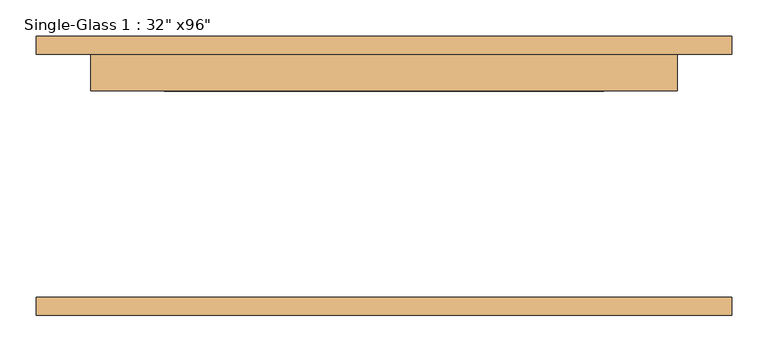
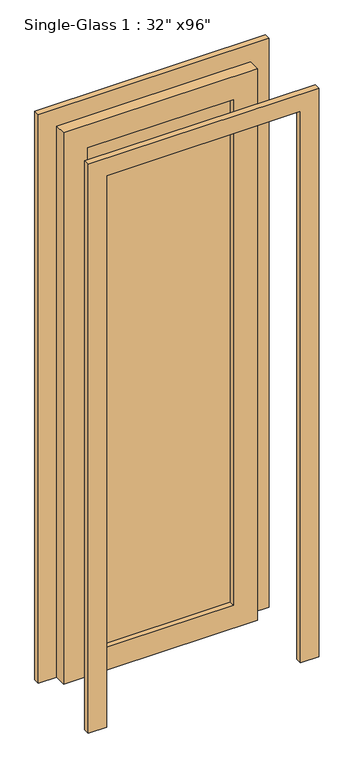
"""IFC4 building model written with IfcOpenShell, lengths in millimetres: door geometry."""

from ifc_helpers import new_model, si_unit, frame, origin, place, context, project, spatial, polyline, outline, extrude, source, transform, mapped, element, save


def door_7e3d8d69(model_context):
    return source(origin(), model_context, "Body", "SweptSolid", [
        extrude(outline(polyline([(2438.4, 406.4), (0.0, 406.4), (0.0, 482.6), (2514.6, 482.6), (2514.6, -482.6), (0.0, -482.6), (0.0, -406.4), (2438.4, -406.4), (2438.4, 406.4)])), frame((0.0, -193.675, 0.0), z_axis=(0.0, 1.0, 0.0), x_axis=(0.0, 0.0, 1.0)), (0.0, 0.0, 1.0), 25.4),
        extrude(outline(polyline([(2438.4, 406.4), (0.0, 406.4), (0.0, 482.6), (2514.6, 482.6), (2514.6, -482.6), (0.0, -482.6), (0.0, -406.4), (2438.4, -406.4), (2438.4, 406.4)])), frame((0.0, 168.275, 0.0), z_axis=(0.0, 1.0, 0.0), x_axis=(0.0, 0.0, 1.0)), (0.0, 0.0, 1.0), 25.4),
        extrude(outline(polyline([(304.8, 139.7), (-304.8, 139.7), (-304.8, 146.05), (304.8, 146.05), (304.8, 139.7)])), frame((0.0, 0.0, 101.6), z_axis=(0.0, 0.0, 1.0), x_axis=(1.0, 0.0, 0.0)), (0.0, 0.0, 1.0), 2235.2),
        extrude(outline(polyline([(2438.4, 406.4), (2438.4, -406.4), (0.0, -406.4), (0.0, 406.4), (2438.4, 406.4)]), holes=[polyline([(2336.8, -304.8), (2336.8, 304.8), (101.6, 304.8), (101.6, -304.8), (2336.8, -304.8)])]), frame((0.0, 117.475, 0.0), z_axis=(0.0, 1.0, 0.0), x_axis=(0.0, 0.0, 1.0)), (0.0, 0.0, 1.0), 50.8),
    ])


if __name__ == "__main__":
    model = new_model("IFC4")
    model_context = context("Model", 3, world=origin())
    ifc_project = project(units=[si_unit("LENGTHUNIT", "METRE", prefix="MILLI")], contexts=[model_context])
    site = spatial("IfcSite", under=ifc_project)
    building = spatial("IfcBuilding", under=site)
    placement = place(None, origin())
    door_shape = door_7e3d8d69(model_context)
    element("IfcDoor", 1, ObjectType="Single-Glass 1 : 32\" x96\"", at=placement, inside=building, context=model_context, shape_type="MappedRepresentation", body=[
        mapped(door_shape, transform((0.0, 0.0, 0.0), x_axis=(1.0, 0.0, 0.0), y_axis=(0.0, 1.0, 0.0), z_axis=(0.0, 0.0, 1.0))),
    ])
    save(model, "model.ifc")

# Revit data of these elements
# Type "Single-Glass 1 : 32\" x96\""
#   Type Mark = "31"
#   Construction Type Id = "MDOOR"
#   Assembly Code = "C1020"
#   Analytic Construction = "Metal"
#   Thickness = 0' - 2"
#   Heat Transfer Coefficient (U) = 3.7021 W/(m²·K)
#   Height = 8' - 0"
#   Rail Width - Base = 0' - 4"
#   Rail Width - Top = 0' - 4"
#   Stile Width - Hinge = 0' - 4"
#   Stile Width - Latch = 0' - 4"
#   Trim Projection Ext = 0' - 1"
#   Trim Projection Int = 0' - 1"
#   Trim Width = 0' - 3"
#   Width = 2' - 8"
#   Door Material = Aluminum
#   Frame Material = Aluminum
#   Visual Light Transmittance = 0
#   Solar Heat Gain Coefficient = 0
#   Function = (empty or 0)
#   Wall Closure = (empty or 0)
# Element 1 (IfcDoor, "Single-Glass 1 : 32\" x96\"")
#   Materials on its faces: "Aluminum", "Glass"
# Materials
#   "Aluminum": class "Metal", colour RGB 226 226 226, transparency 0, Description = "Aluminum 6061", Cost = 0
#   "Glass": class "Glass", colour RGB 142 168 196, transparency 0.75, Description = "Soda Lime Glass", Cost = 0
